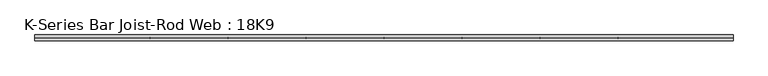
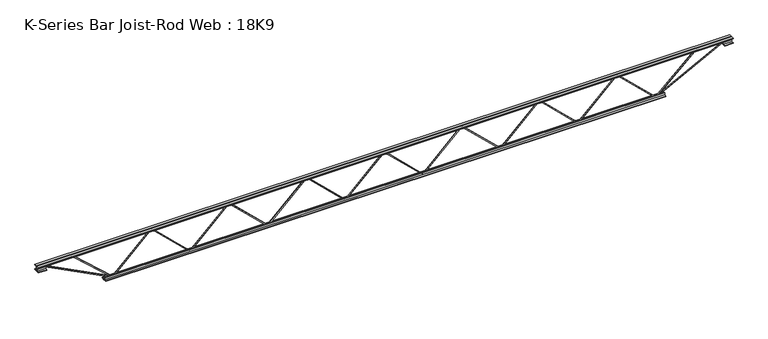
"""IFC4 building model written with IfcOpenShell, lengths in millimetres: beam geometry, K-Series Bar Joist-Rod Web : 18K9."""

from ifc_helpers import new_model, si_unit, frame, origin, place, context, project, spatial, polyline, outline, extrude, source, transform, mapped, element, save


def k_series_bar_joist_rod_web_18k9_858c7c49(model_context):
    return source(origin(), model_context, "Body", "SweptSolid", [
        extrude(outline(polyline([(-217.4875, 1404.2571429), (-227.0125, 1404.2571429), (-227.0125, 1409.3519885), (217.4875, 1871.0877028), (217.4875, 1873.5980115), (-227.0125, 2335.3337258), (-227.0125, 2340.4285714), (-217.4875, 2340.4285714), (-217.4875, 2339.173417), (227.0125, 1877.4377028), (227.0125, 1867.2480115), (-217.4875, 1405.5122972), (-217.4875, 1404.2571429)])), frame((0.0, -4.7625, 0.0), z_axis=(0.0, 1.0, 0.0), x_axis=(0.0, 0.0, 1.0)), (0.0, 0.0, 1.0), 9.525),
        extrude(outline(polyline([(-217.4875, 468.0857143), (-227.0125, 468.0857143), (-227.0125, 473.1805599), (217.4875, 934.9162742), (217.4875, 937.426583), (-227.0125, 1399.1622972), (-227.0125, 1404.2571429), (-217.4875, 1404.2571429), (-217.4875, 1403.0019885), (227.0125, 941.2662742), (227.0125, 931.076583), (-217.4875, 469.3408687), (-217.4875, 468.0857143)])), frame((0.0, -4.7625, 0.0), z_axis=(0.0, 1.0, 0.0), x_axis=(0.0, 0.0, 1.0)), (0.0, 0.0, 1.0), 9.525),
        extrude(outline(polyline([(-217.4875, -468.0857143), (-227.0125, -468.0857143), (-227.0125, -462.9908687), (217.4875, -1.2551544), (217.4875, 1.2551544), (-227.0125, 462.9908687), (-227.0125, 468.0857143), (-217.4875, 468.0857143), (-217.4875, 466.8305599), (227.0125, 5.0948456), (227.0125, -5.0948456), (-217.4875, -466.8305599), (-217.4875, -468.0857143)])), frame((0.0, -4.7625, 0.0), z_axis=(0.0, 1.0, 0.0), x_axis=(0.0, 0.0, 1.0)), (0.0, 0.0, 1.0), 9.525),
        extrude(outline(polyline([(-217.4875, -1404.2571429), (-227.0125, -1404.2571429), (-227.0125, -1399.1622972), (217.4875, -937.426583), (217.4875, -934.9162742), (-227.0125, -473.1805599), (-227.0125, -468.0857143), (-217.4875, -468.0857143), (-217.4875, -469.3408687), (227.0125, -931.076583), (227.0125, -941.2662742), (-217.4875, -1403.0019885), (-217.4875, -1404.2571429)])), frame((0.0, -4.7625, 0.0), z_axis=(0.0, 1.0, 0.0), x_axis=(0.0, 0.0, 1.0)), (0.0, 0.0, 1.0), 9.525),
        extrude(outline(polyline([(-217.4875, -2340.4285714), (-227.0125, -2340.4285714), (-227.0125, -2335.3337258), (217.4875, -1873.5980115), (217.4875, -1871.0877028), (-227.0125, -1409.3519885), (-227.0125, -1404.2571429), (-217.4875, -1404.2571429), (-217.4875, -1405.5122972), (227.0125, -1867.2480115), (227.0125, -1877.4377028), (-217.4875, -2339.173417), (-217.4875, -2340.4285714)])), frame((0.0, -4.7625, 0.0), z_axis=(0.0, 1.0, 0.0), x_axis=(0.0, 0.0, 1.0)), (0.0, 0.0, 1.0), 9.525),
        extrude(outline(polyline([(-217.4875, 2340.4285714), (-227.0125, 2340.4285714), (-227.0125, 2345.523417), (217.4875, 2807.2591313), (217.4875, 2809.7694401), (-227.0125, 3271.5051544), (-227.0125, 3276.6), (-217.4875, 3276.6), (-217.4875, 3275.3448456), (227.0125, 2813.6091313), (227.0125, 2803.4194401), (-217.4875, 2341.6837258), (-217.4875, 2340.4285714)])), frame((0.0, -4.7625, 0.0), z_axis=(0.0, 1.0, 0.0), x_axis=(0.0, 0.0, 1.0)), (0.0, 0.0, 1.0), 9.525),
        extrude(outline(polyline([(-217.4875, -3276.6), (-227.0125, -3276.6), (-227.0125, -3271.5051544), (217.4875, -2809.7694401), (217.4875, -2807.2591313), (-227.0125, -2345.523417), (-227.0125, -2340.4285714), (-217.4875, -2340.4285714), (-217.4875, -2341.6837258), (227.0125, -2803.4194401), (227.0125, -2813.6091313), (-217.4875, -3275.3448456), (-217.4875, -3276.6)])), frame((0.0, -4.7625, 0.0), z_axis=(0.0, 1.0, 0.0), x_axis=(0.0, 0.0, 1.0)), (0.0, 0.0, 1.0), 9.525),
        extrude(outline(polyline([(4.7625, 228.6), (36.5125, 228.6), (36.5125, 222.25), (11.1125, 222.25), (11.1125, 196.85), (4.7625, 196.85), (4.7625, 228.6)])), frame((-4191.0, 0.0, 0.0), z_axis=(1.0, 0.0, 0.0), x_axis=(0.0, 1.0, 0.0)), (0.0, 0.0, 1.0), 8382.0),
        extrude(outline(polyline([(-4.7625, 228.6), (-4.7625, 196.85), (-11.1125, 196.85), (-11.1125, 222.25), (-36.5125, 222.25), (-36.5125, 228.6), (-4.7625, 228.6)])), frame((-4191.0, 0.0, 0.0), z_axis=(1.0, 0.0, 0.0), x_axis=(0.0, 1.0, 0.0)), (0.0, 0.0, 1.0), 8382.0),
        extrude(outline(polyline([(-4.7625, 165.1), (-36.5125, 165.1), (-36.5125, 171.45), (-11.1125, 171.45), (-11.1125, 196.85), (-4.7625, 196.85), (-4.7625, 165.1)])), frame((-4191.0, 0.0, 0.0), z_axis=(1.0, 0.0, 0.0), x_axis=(0.0, 1.0, 0.0)), (0.0, 0.0, 1.0), 101.6),
        extrude(outline(polyline([(36.5125, 165.1), (4.7625, 165.1), (4.7625, 196.85), (11.1125, 196.85), (11.1125, 171.45), (36.5125, 171.45), (36.5125, 165.1)])), frame((-4191.0, 0.0, 0.0), z_axis=(1.0, 0.0, 0.0), x_axis=(0.0, 1.0, 0.0)), (0.0, 0.0, 1.0), 101.6),
        extrude(outline(polyline([(4.7625, 165.1), (4.7625, 196.85), (11.1125, 196.85), (11.1125, 171.45), (36.5125, 171.45), (36.5125, 165.1), (4.7625, 165.1)])), frame((4089.4, 0.0, 0.0), z_axis=(1.0, 0.0, 0.0), x_axis=(0.0, 1.0, 0.0)), (0.0, 0.0, 1.0), 101.6),
        extrude(outline(polyline([(-4.7625, 165.1), (-36.5125, 165.1), (-36.5125, 171.45), (-11.1125, 171.45), (-11.1125, 196.85), (-4.7625, 196.85), (-4.7625, 165.1)])), frame((4089.4, 0.0, 0.0), z_axis=(1.0, 0.0, 0.0), x_axis=(0.0, 1.0, 0.0)), (0.0, 0.0, 1.0), 101.6),
        extrude(outline(polyline([(4.7625, -228.6), (4.7625, -196.85), (11.1125, -196.85), (11.1125, -222.25), (36.5125, -222.25), (36.5125, -228.6), (4.7625, -228.6)])), frame((-3378.2, 0.0, 0.0), z_axis=(1.0, 0.0, 0.0), x_axis=(0.0, 1.0, 0.0)), (0.0, 0.0, 1.0), 6756.4),
        extrude(outline(polyline([(-4.7625, -228.6), (-36.5125, -228.6), (-36.5125, -222.25), (-11.1125, -222.25), (-11.1125, -196.85), (-4.7625, -196.85), (-4.7625, -228.6)])), frame((-3378.2, 0.0, 0.0), z_axis=(1.0, 0.0, 0.0), x_axis=(0.0, 1.0, 0.0)), (0.0, 0.0, 1.0), 6756.4),
        extrude(outline(polyline([(0.0, -9.525), (0.0, 0.0), (914.4881902, 0.0), (914.4881902, -9.525), (0.0, -9.525)])), frame((-4091.582602, 4.7625, 192.6170749), z_axis=(0.45828913319472664, 0.0, 0.8888031674086373), x_axis=(0.8888031674086373, 0.0, -0.45828913319472664)), (0.0, 0.0, 1.0), 9.525),
        extrude(outline(polyline([(0.0, -9.525), (0.0, 0.0), (628.2905744, 0.0), (628.2905744, -9.525), (0.0, -9.525)])), frame((-3747.8625306, 4.7625, 193.3018675), z_axis=(0.667048046009021, 0.0, 0.745014700737876), x_axis=(0.745014700737876, 0.0, -0.667048046009021)), (0.0, 0.0, 1.0), 9.525),
        extrude(outline(polyline([(0.0, -9.525), (0.0, 0.0), (914.4881902, 0.0), (914.4881902, -9.525), (0.0, -9.525)])), frame((4091.582602, -4.7625, 192.6170749), z_axis=(-0.4582891331947151, 0.0, 0.8888031674086432), x_axis=(-0.8888031674086432, 0.0, -0.4582891331947151)), (0.0, 0.0, 1.0), 9.525),
        extrude(outline(polyline([(0.0, -9.525), (0.0, 0.0), (628.2905744, 0.0), (628.2905744, -9.525), (0.0, -9.525)])), frame((3747.8625306, -4.7625, 193.3018675), z_axis=(-0.6670480460090169, 0.0, 0.7450147007378798), x_axis=(-0.7450147007378798, 0.0, -0.6670480460090169)), (0.0, 0.0, 1.0), 9.525),
    ])


if __name__ == "__main__":
    model = new_model("IFC4")
    model_context = context("Model", 3, world=origin())
    ifc_project = project(units=[si_unit("LENGTHUNIT", "METRE", prefix="MILLI")], contexts=[model_context])
    site = spatial("IfcSite", under=ifc_project)
    building = spatial("IfcBuilding", under=site)
    placement = place(None, origin())
    k_series_bar_joist_rod_web_18k9_shape = k_series_bar_joist_rod_web_18k9_858c7c49(model_context)
    element("IfcBeam", 1, ObjectType="K-Series Bar Joist-Rod Web : 18K9", at=placement, inside=building, context=model_context, shape_type="MappedRepresentation", body=[
        mapped(k_series_bar_joist_rod_web_18k9_shape, transform((0.0, 0.0, 0.0), x_axis=(1.0, 0.0, 0.0), y_axis=(0.0, 1.0, 0.0), z_axis=(0.0, 0.0, 1.0))),
    ])
    save(model, "model.ifc")

# Revit data of these elements
# Type "K-Series Bar Joist-Rod Web : 18K9"
#   Assembly Code = "B1010350"
#   Wt = 10.2
#   Web Thickness = 0' - 0 3/8"
#   Start Offset [instance default] = 0' - 0"
#   Start Extension [instance default] = 0' - 0"
#   Seat Length = 0' - 4"
#   Seat Depth = 0' - 2 1/2"
#   PanelArrayLength [instance default] = 18' - 0"
#   Panel [instance default] = 3' - 0"
#   End Offset [instance default] = 0' - 0"
#   End Extension [instance default] = 0' - 0"
#   End Panel = 3' - 0"
#   Cord Leg = 0' - 1 1/4"
#   Chord Thickness = 0' - 0 1/4"
#   Length [instance default] = 24' - 0"
#   Depth = 1' - 6"
#   PanelArrayNum [instance default] = 6
#   Structural Material = none
# Element 1 (IfcBeam, "K-Series Bar Joist-Rod Web : 18K9")
#   PanelArrayLength = 21' - 6"
#   Panel = 3' - 0.85714"
#   PanelArrayNum = 7
